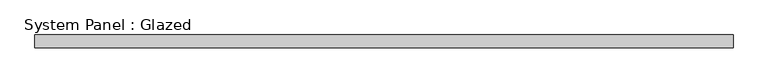
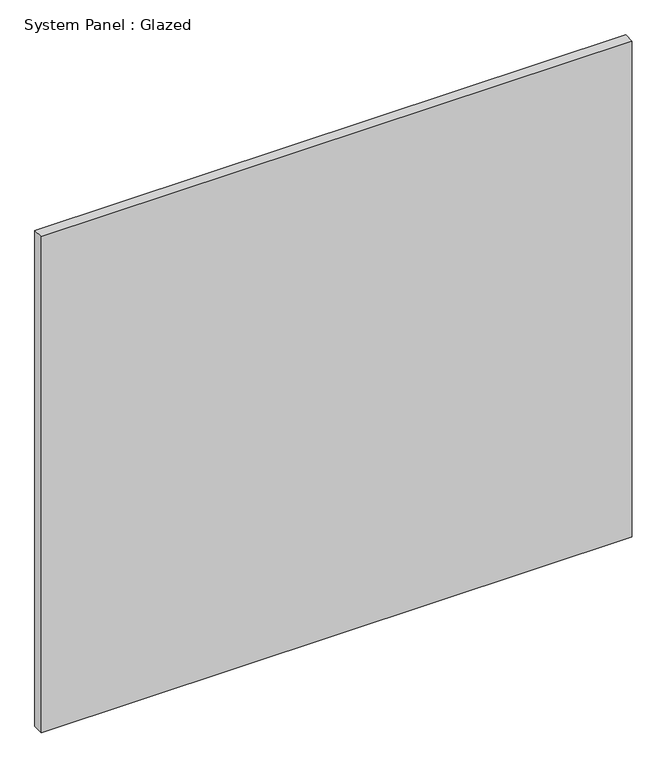
"""IFC4 building model written with IfcOpenShell, lengths in millimetres: plate geometry, System Panel : Glazed."""

from ifc_helpers import new_model, si_unit, origin, origin_with_axes, place, context, project, spatial, polyline, outline, extrude, source, transform, mapped, element, save


def system_panel_glazed_cc8ec8cc(model_context):
    return source(origin(), model_context, "Body", "SweptSolid", [
        extrude(outline(polyline([(676.3401298, 24.5), (-676.3401298, 24.5), (-676.3401298, 49.5), (676.3401298, 49.5), (676.3401298, 24.5)])), origin_with_axes(), (0.0, 0.0, 1.0), 1200.0),
    ])


if __name__ == "__main__":
    model = new_model("IFC4")
    model_context = context("Model", 3, world=origin())
    ifc_project = project(units=[si_unit("LENGTHUNIT", "METRE", prefix="MILLI")], contexts=[model_context])
    site = spatial("IfcSite", under=ifc_project)
    building = spatial("IfcBuilding", under=site)
    placement = place(None, origin())
    system_panel_glazed_shape = system_panel_glazed_cc8ec8cc(model_context)
    element("IfcPlate", 1, ObjectType="System Panel : Glazed", at=placement, inside=building, context=model_context, shape_type="MappedRepresentation", body=[
        mapped(system_panel_glazed_shape, transform((0.0, 0.0, 0.0), x_axis=(1.0, 0.0, 0.0), y_axis=(0.0, 1.0, 0.0), z_axis=(0.0, 0.0, 1.0))),
    ])
    save(model, "model.ifc")

# Revit data of these elements
# Element 1 (IfcPlate, "System Panel : Glazed")
#   Materials on its faces: "Glass"
# Materials
#   "Glass": class "Glass", colour RGB 218 227 224, transparency 0.85, Description = "Soda Lime Glass", Cost = 0
